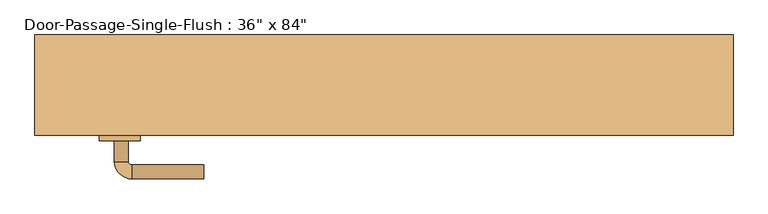
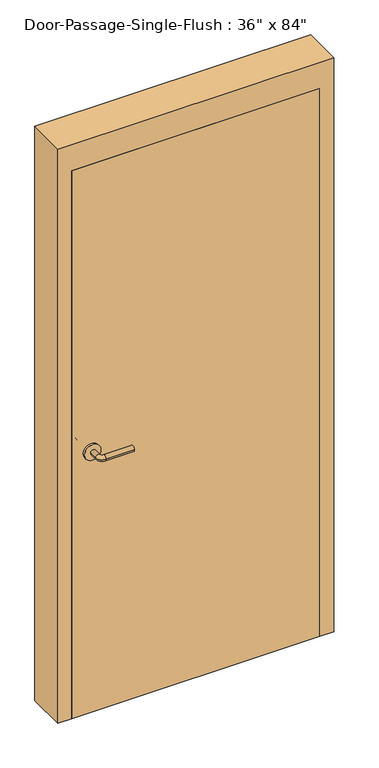
"""IFC4 building model written with IfcOpenShell, lengths in millimetres: door geometry."""

import ifcopenshell
import ifcopenshell.guid

model = None  # the IFC model being written
_history = None  # IfcOwnerHistory: only IFC2X3 demands one
_inside = {}  # id of a spatial element -> (the spatial element, [elements in it])
_under = {}  # id of a project, library or spatial element -> (it, [spatial elements below it])
_declared = {}  # id of a project -> (the project, [libraries it declares])
_typed = {}  # id of a type object -> (the type object, [elements of that type])
_made_of = {}  # id of a material, layer set ... -> (it, [elements and type objects made of it])


def new_model(schema):
    """Start an empty IFC model of exactly this schema.

    Asked for "IFC4X3", IfcOpenShell would pick the latest addendum, in which some entities
    have other attributes; the version numbers below select the first issue.
    IFC2X3 requires an IfcOwnerHistory on every rooted entity: one is made here for all.
    """
    global model, _history
    if schema == "IFC4X3":
        model = ifcopenshell.file(schema_version=(4, 3, 0, 0))
    else:
        model = ifcopenshell.file(schema=schema)
    _inside.clear()
    _under.clear()
    _declared.clear()
    _typed.clear()
    _made_of.clear()
    _history = None
    if model.schema == "IFC2X3":
        org = make("IfcOrganization", Name="unknown")
        user = make(
            "IfcPersonAndOrganization",
            ThePerson=make("IfcPerson", FamilyName="unknown"),
            TheOrganization=org,
        )
        app = make(
            "IfcApplication",
            ApplicationDeveloper=org,
            Version="unknown",
            ApplicationFullName="unknown",
            ApplicationIdentifier="unknown",
        )
        _history = make(
            "IfcOwnerHistory",
            OwningUser=user,
            OwningApplication=app,
            ChangeAction="ADDED",
            CreationDate=0,
        )
    return model


def make(cls, **values):
    """One entity of the class cls with the attributes given. An attribute that is None is left unset."""
    return model.create_entity(
        cls, **{name: value for name, value in values.items() if value is not None}
    )


def rooted(cls, **values):
    """An entity with a GlobalId (a new one), such as an element, a storey or a relation."""
    return make(cls, GlobalId=ifcopenshell.guid.new(), OwnerHistory=_history, **values)


def si_unit(unit_type, name, prefix=None):
    """IfcSIUnit, for example si_unit("LENGTHUNIT", "METRE", prefix="MILLI")."""
    return make("IfcSIUnit", UnitType=unit_type, Prefix=prefix, Name=name)


def assignment(units):
    """IfcUnitAssignment: the units of a project."""
    return None if units is None else make("IfcUnitAssignment", Units=units)


def point(xyz):
    """IfcCartesianPoint."""
    return None if xyz is None else make("IfcCartesianPoint", Coordinates=xyz)


def direction(xyz):
    """IfcDirection."""
    return None if xyz is None else make("IfcDirection", DirectionRatios=xyz)


def frame(location, z_axis=None, x_axis=None):
    """IfcAxis2Placement3D, a coordinate frame: its origin and axes. An axis left out is left unset."""
    return make(
        "IfcAxis2Placement3D",
        Location=point(location),
        Axis=direction(z_axis),
        RefDirection=direction(x_axis),
    )


def frame_2d(location, x_axis=None):
    """IfcAxis2Placement2D, a coordinate frame in the plane: its origin and x axis."""
    return make(
        "IfcAxis2Placement2D", Location=point(location), RefDirection=direction(x_axis)
    )


def origin():
    """The frame at (0, 0, 0) with its axes left unset."""
    return frame((0.0, 0.0, 0.0))


def origin_with_axes():
    """The frame at (0, 0, 0) with the z axis (0, 0, 1) and the x axis (1, 0, 0) written out."""
    return frame((0.0, 0.0, 0.0), z_axis=(0.0, 0.0, 1.0), x_axis=(1.0, 0.0, 0.0))


def place(relative_to, where):
    """IfcLocalPlacement: puts the frame where relative to a parent placement (None: the world)."""
    return make(
        "IfcLocalPlacement", PlacementRelTo=relative_to, RelativePlacement=where
    )


def context(
    kind, dimensions, precision=None, world=None, true_north=None, identifier=None
):
    """IfcGeometricRepresentationContext, for example the 3D "Model" context."""
    return make(
        "IfcGeometricRepresentationContext",
        ContextIdentifier=identifier,
        ContextType=kind,
        CoordinateSpaceDimension=dimensions,
        Precision=precision,
        WorldCoordinateSystem=world,
        TrueNorth=true_north,
    )


def project(units=None, contexts=None):
    """IfcProject with its units and contexts."""
    return rooted(
        "IfcProject",
        Name="project",
        RepresentationContexts=contexts,
        UnitsInContext=assignment(units),
    )


def spatial(cls, under=None, at=None, **own):
    """A site, building, storey or space (cls), placed at a placement, below another one or the project."""
    s = rooted(cls, ObjectPlacement=at, **own)
    if under is not None:
        _under.setdefault(under.id(), (under, []))[1].append(s)
    return s


def polyline(points):
    """IfcPolyline through the points."""
    return make("IfcPolyline", Points=[point(p) for p in points])


def circle_curve(where, radius):
    """IfcCircle in the frame where."""
    return make("IfcCircle", Position=where, Radius=radius)


def ellipse_curve(where, semi_axis1, semi_axis2):
    """IfcEllipse in the frame where."""
    return make(
        "IfcEllipse", Position=where, SemiAxis1=semi_axis1, SemiAxis2=semi_axis2
    )


def trimmed(basis, trim1, trim2, sense, master):
    """IfcTrimmedCurve: the piece of a basis curve between two trims."""
    return make(
        "IfcTrimmedCurve",
        BasisCurve=basis,
        Trim1=trim1,
        Trim2=trim2,
        SenseAgreement=sense,
        MasterRepresentation=master,
    )


def segment(curve, same_sense, transition):
    """IfcCompositeCurveSegment."""
    return make(
        "IfcCompositeCurveSegment",
        Transition=transition,
        SameSense=same_sense,
        ParentCurve=curve,
    )


def composite_curve(segments, self_intersect=None):
    """IfcCompositeCurve: segments joined end to end."""
    return make("IfcCompositeCurve", Segments=segments, SelfIntersect=self_intersect)


def outline(outer, holes=None, kind="AREA"):
    """IfcArbitraryClosedProfileDef: a profile drawn as a closed curve; with holes, ...WithVoids."""
    if holes is None:
        return make("IfcArbitraryClosedProfileDef", ProfileType=kind, OuterCurve=outer)
    return make(
        "IfcArbitraryProfileDefWithVoids",
        ProfileType=kind,
        OuterCurve=outer,
        InnerCurves=holes,
    )


def extrude(swept, where, along, depth):
    """IfcExtrudedAreaSolid: the profile swept, set in the frame where, extruded along a direction by depth."""
    return make(
        "IfcExtrudedAreaSolid",
        SweptArea=swept,
        Position=where,
        ExtrudedDirection=direction(along),
        Depth=depth,
    )


def faces_of(points, faces, orient=None, outer=None):
    """IfcFace entities. A face is a list of loops; a loop is a list of indices into points, from 0.

    orient and outer hold one flag for each loop. By default every Orientation is true, the
    first loop of a face is its IfcFaceOuterBound and the others are IfcFaceBound.
    """
    made = []
    for i, loops in enumerate(faces):
        bounds = []
        for j, loop in enumerate(loops):
            is_outer = j == 0 if outer is None else outer[i][j]
            bounds.append(
                make(
                    "IfcFaceOuterBound" if is_outer else "IfcFaceBound",
                    Bound=make("IfcPolyLoop", Polygon=[points[k] for k in loop]),
                    Orientation=True if orient is None else orient[i][j],
                )
            )
        made.append(make("IfcFace", Bounds=bounds))
    return made


def faceted_brep(points, faces, orient=None, outer=None, voids=None):
    """IfcFacetedBrep: a solid bounded by flat faces; with voids (closed shells), ...WithVoids."""
    shared = [point(p) for p in points]
    hull = make("IfcClosedShell", CfsFaces=faces_of(shared, faces, orient, outer))
    if voids is None:
        return make("IfcFacetedBrep", Outer=hull)
    return make(
        "IfcFacetedBrepWithVoids",
        Outer=hull,
        Voids=[
            make(cls, CfsFaces=faces_of(shared, fs, o, b)) for cls, fs, o, b in voids
        ],
    )


def shape(context_of_items, identifier, shape_type, items):
    """IfcShapeRepresentation: the items that make up one representation, for example the "Body"."""
    return make(
        "IfcShapeRepresentation",
        ContextOfItems=context_of_items,
        RepresentationIdentifier=identifier,
        RepresentationType=shape_type,
        Items=items,
    )


def source(mapping_origin, context_of_items, identifier, shape_type, items):
    """IfcRepresentationMap: a shape defined once, which mapped items show again and again."""
    return make(
        "IfcRepresentationMap",
        MappingOrigin=mapping_origin,
        MappedRepresentation=shape(context_of_items, identifier, shape_type, items),
    )


def transform(
    local_origin,
    x_axis=None,
    y_axis=None,
    z_axis=None,
    scale=None,
    scale2=None,
    scale3=None,
    uniform=True,
):
    """IfcCartesianTransformationOperator3D, or its non-uniform kind. x_axis, y_axis, z_axis: its Axis1, 2, 3."""
    if uniform:
        return make(
            "IfcCartesianTransformationOperator3D",
            Axis1=direction(x_axis),
            Axis2=direction(y_axis),
            LocalOrigin=point(local_origin),
            Scale=scale,
            Axis3=direction(z_axis),
        )
    return make(
        "IfcCartesianTransformationOperator3DnonUniform",
        Axis1=direction(x_axis),
        Axis2=direction(y_axis),
        LocalOrigin=point(local_origin),
        Scale=scale,
        Axis3=direction(z_axis),
        Scale2=scale2,
        Scale3=scale3,
    )


def mapped(mapping_source, mapping_target):
    """IfcMappedItem: shows the shape of a source again, moved by a transform."""
    return make(
        "IfcMappedItem", MappingSource=mapping_source, MappingTarget=mapping_target
    )


def made_of(thing, what):
    """Note that an element or type object is made of a material, layer set ...; save() writes the relation."""
    if what is not None:
        _made_of.setdefault(what.id(), (what, []))[1].append(thing)
    return thing


def element(
    cls,
    number,
    at=None,
    inside=None,
    cuts=None,
    type_object=None,
    material=None,
    context=None,
    identifier="Body",
    shape_type=None,
    held_by="IfcProductDefinitionShape",
    body=None,
    shapes=None,
    **own,
):
    """One element of the class cls, such as IfcWall. Its Tag is "e" and its number.

    at: its placement. inside: the storey or other place that contains it. cuts: it is an
    opening in that element (IfcRelVoidsElement). A single representation is given by context,
    identifier, shape_type and body (its items); several are given by shapes. held_by: the class
    of the entity that holds the representations. save() writes the other relations.
    """
    e = rooted(cls, Tag="e%d" % number, ObjectPlacement=at, **own)
    if body is not None:
        shapes = [shape(context, identifier, shape_type, body)]
    if shapes is not None:
        e.Representation = make(held_by, Representations=shapes)
    if inside is not None:
        _inside.setdefault(inside.id(), (inside, []))[1].append(e)
    if cuts is not None:
        rooted(
            "IfcRelVoidsElement", RelatingBuildingElement=cuts, RelatedOpeningElement=e
        )
    if type_object is not None:
        _typed.setdefault(type_object.id(), (type_object, []))[1].append(e)
    return made_of(e, material)


def aggregate(whole, parts):
    """IfcRelAggregates: a whole, such as a stair, and the parts it consists of."""
    return rooted("IfcRelAggregates", RelatingObject=whole, RelatedObjects=parts)


def save(model, path):
    """Write the relations noted so far, then the file.

    IfcRelAggregates (storeys below a building ...), IfcRelContainedInSpatialStructure (elements
    in a storey), IfcRelDefinesByType, IfcRelAssociatesMaterial and IfcRelDeclares: one each for
    every whole, place, type object, material and project.
    """
    for whole, parts in _under.values():
        aggregate(whole, parts)
    for where, things in _inside.values():
        rooted(
            "IfcRelContainedInSpatialStructure",
            RelatedElements=things,
            RelatingStructure=where,
        )
    for kind, things in _typed.values():
        rooted("IfcRelDefinesByType", RelatedObjects=things, RelatingType=kind)
    for what, things in _made_of.values():
        rooted("IfcRelAssociatesMaterial", RelatedObjects=things, RelatingMaterial=what)
    for by, libraries in _declared.values():
        rooted("IfcRelDeclares", RelatingContext=by, RelatedDefinitions=libraries)
    model.write(path)


def plane_surface(at):
    """IfcPlane: the flat surface through the origin of the frame at, square to its z axis."""
    return make("IfcPlane", Position=at)


def cylinder_surface(at, radius):
    """IfcCylindricalSurface: all points at the distance radius from the z axis of the frame at."""
    return make("IfcCylindricalSurface", Position=at, Radius=radius)


def revolved_surface(curve, axis_point, axis_direction):
    """IfcSurfaceOfRevolution: the curve turned about the line through axis_point along axis_direction."""
    return make(
        "IfcSurfaceOfRevolution",
        SweptCurve=make("IfcArbitraryOpenProfileDef", ProfileType="CURVE", Curve=curve),
        AxisPosition=make("IfcAxis1Placement", Location=point(axis_point), Axis=direction(axis_direction)),
    )


def advanced_brep(points, edges, surfaces, faces):
    """IfcAdvancedBrep: a solid bounded by faces that lie on surfaces and meet in shared edges.

    An edge is (start, end): straight between two places in points (the first is 0);
    or (start, end, curve); or (start, end, curve, False) where it runs against its curve.
    A face is (place in surfaces, loops), or (place, loops, False) where it looks against
    its surface's normal. A loop lists edges by number (the first is 1), with a minus sign
    where the edge is run from its end to its start. The first loop is the outer one.
    """
    corners = [point(p) for p in points]
    vertices = [make("IfcVertexPoint", VertexGeometry=c) for c in corners]
    made = []
    for start, end, *more in edges:
        made.append(
            make(
                "IfcEdgeCurve",
                EdgeStart=vertices[start],
                EdgeEnd=vertices[end],
                EdgeGeometry=more[0] if more else make("IfcPolyline", Points=[corners[start], corners[end]]),
                SameSense=more[1] if len(more) > 1 else True,
            )
        )
    hull = []
    for where, loops, *sense in faces:
        bounds = []
        for j, loop in enumerate(loops):
            ring = [make("IfcOrientedEdge", EdgeElement=made[abs(k) - 1], Orientation=k > 0) for k in loop]
            bounds.append(
                make(
                    "IfcFaceOuterBound" if j == 0 else "IfcFaceBound",
                    Bound=make("IfcEdgeLoop", EdgeList=ring),
                    Orientation=True,
                )
            )
        hull.append(make("IfcAdvancedFace", Bounds=bounds, FaceSurface=surfaces[where], SameSense=sense[0] if sense else True))
    return make("IfcAdvancedBrep", Outer=make("IfcClosedShell", CfsFaces=hull))


def door_36f17018(model_context):
    return source(origin(), model_context, "Body", "SolidModel", [
        advanced_brep(
        [(-392.190625, -23.75, 1016.0), (-372.190625, -23.75, 1016.0), (-392.190625, 6.25, 1016.0), (-372.190625, 6.25, 1016.0), (-367.190625, 11.25, 1016.0), (-367.190625, 31.25, 1016.0), (-262.190625, 31.25, 1016.0), (-262.190625, 11.25, 1016.0)],
        [
            (0, 1, circle_curve(frame((-382.190625, -23.75, 1016.0), z_axis=(0.0, -1.0, 0.0), x_axis=(1.0, 0.0, 0.0)), 10.0)),
            (1, 0, circle_curve(frame((-382.190625, -23.75, 1016.0), z_axis=(0.0, -1.0, 0.0), x_axis=(1.0, 0.0, 0.0)), 10.0)),
            (0, 2),
            (2, 3, circle_curve(frame((-382.190625, 6.25, 1016.0), z_axis=(0.0, -1.0, 0.0), x_axis=(1.0, 0.0, 0.0)), 10.0)),
            (3, 1),
            (3, 2, circle_curve(frame((-382.190625, 6.25, 1016.0), z_axis=(0.0, -1.0, 0.0), x_axis=(1.0, 0.0, 0.0)), 10.0)),
            (4, 3, circle_curve(frame((-367.190625, 6.25, 1016.0), z_axis=(0.0, 0.0, 1.0), x_axis=(-1.0, 0.0, 0.0)), 5.0)),
            (2, 5, circle_curve(frame((-367.190625, 6.25, 1016.0), z_axis=(0.0, 0.0, -1.0), x_axis=(-1.0, 0.0, 0.0)), 25.0)),
            (5, 4, circle_curve(frame((-367.190625, 21.25, 1016.0), z_axis=(-1.0, 0.0, 0.0), x_axis=(0.0, -1.0, 0.0)), 10.0)),
            (4, 5, circle_curve(frame((-367.190625, 21.25, 1016.0), z_axis=(-1.0, 0.0, 0.0), x_axis=(0.0, -1.0, 0.0)), 10.0)),
            (6, 7, circle_curve(frame((-262.190625, 21.25, 1016.0), z_axis=(1.0, 0.0, 0.0), x_axis=(0.0, -1.0, 0.0)), 10.0)),
            (7, 6, circle_curve(frame((-262.190625, 21.25, 1016.0), z_axis=(1.0, 0.0, 0.0), x_axis=(0.0, -1.0, 0.0)), 10.0)),
            (5, 6),
            (7, 4),
        ],
        [
            plane_surface(frame((-382.190625, -23.75, 1016.0), z_axis=(0.0, -1.0, 0.0), x_axis=(0.0, 0.0, 1.0))),
            cylinder_surface(frame((-382.190625, -23.75, 1016.0), z_axis=(0.0, -1.0, 0.0), x_axis=(1.0, 0.0, 0.0)), 10.0),
            revolved_surface(trimmed(ellipse_curve(frame((-382.190625, 6.25, 1016.0), z_axis=(0.0, -1.0, 0.0), x_axis=(1.0, 0.0, 0.0)), 10.0, 10.0), [point((-392.190625, 6.25, 1016.0))], [point((-372.190625, 6.25, 1016.0))], True, "CARTESIAN"), (-367.190625, 6.25, 1016.0), (0.0, 0.0, -1.0)),
            revolved_surface(trimmed(ellipse_curve(frame((-382.190625, 6.25, 1016.0), z_axis=(0.0, -1.0, 0.0), x_axis=(1.0, 0.0, 0.0)), 10.0, 10.0), [point((-372.190625, 6.25, 1016.0))], [point((-392.190625, 6.25, 1016.0))], True, "CARTESIAN"), (-367.190625, 6.25, 1016.0), (0.0, 0.0, -1.0)),
            plane_surface(frame((-262.190625, 21.25, 1016.0), z_axis=(1.0, 0.0, 0.0), x_axis=(0.0, 0.0, 1.0))),
            cylinder_surface(frame((-367.190625, 21.25, 1016.0), z_axis=(-1.0, 0.0, 0.0), x_axis=(0.0, -1.0, 0.0)), 10.0),
        ],
        [
            (0, [[1, 2]]),
            (1, [[-1, 3, 4, 5]]),
            (1, [[-2, -5, 6, -3]]),
            (2, [[7, -4, 8, 9]]),
            (3, [[-8, -6, -7, 10]]),
            (4, [[11, 12]]),
            (5, [[-9, 13, -12, 14]]),
            (5, [[-10, -14, -11, -13]]),
        ],
    ),
        extrude(outline(composite_curve([segment(trimmed(circle_curve(frame_2d((1016.0, -384.690625)), 30.0), [point((1016.0, -414.690625))], [point((1016.0, -354.690625))], False, "CARTESIAN"), True, "CONTINUOUS"), segment(trimmed(circle_curve(frame_2d((1016.0, -384.690625)), 30.0), [point((1016.0, -354.690625))], [point((1016.0, -414.690625))], False, "CARTESIAN"), True, "CONTINUOUS")], self_intersect=False)), frame((0.0, -31.75, 0.0), z_axis=(0.0, 1.0, 0.0), x_axis=(0.0, 0.0, 1.0)), (0.0, 0.0, 1.0), 8.0),
        advanced_brep(
        [(-392.190625, -84.2, 1016.0), (-372.190625, -84.2, 1016.0), (-372.190625, -114.2, 1016.0), (-392.190625, -114.2, 1016.0), (-367.190625, -119.2, 1016.0), (-367.190625, -139.2, 1016.0), (-262.190625, -139.2, 1016.0), (-262.190625, -119.2, 1016.0)],
        [
            (0, 1, circle_curve(frame((-382.190625, -84.2, 1016.0), z_axis=(0.0, 1.0, 0.0), x_axis=(1.0, 0.0, 0.0)), 10.0)),
            (1, 0, circle_curve(frame((-382.190625, -84.2, 1016.0), z_axis=(0.0, 1.0, 0.0), x_axis=(1.0, 0.0, 0.0)), 10.0)),
            (1, 2),
            (2, 3, circle_curve(frame((-382.190625, -114.2, 1016.0), z_axis=(0.0, 1.0, 0.0), x_axis=(1.0, 0.0, 0.0)), 10.0)),
            (3, 0),
            (3, 2, circle_curve(frame((-382.190625, -114.2, 1016.0), z_axis=(0.0, 1.0, 0.0), x_axis=(1.0, 0.0, 0.0)), 10.0)),
            (4, 5, circle_curve(frame((-367.190625, -129.2, 1016.0), z_axis=(-1.0, 0.0, 0.0), x_axis=(0.0, 1.0, 0.0)), 10.0)),
            (5, 3, circle_curve(frame((-367.190625, -114.2, 1016.0), z_axis=(0.0, 0.0, -1.0), x_axis=(-1.0, 0.0, 0.0)), 25.0)),
            (2, 4, circle_curve(frame((-367.190625, -114.2, 1016.0), z_axis=(0.0, 0.0, 1.0), x_axis=(-1.0, 0.0, 0.0)), 5.0)),
            (5, 4, circle_curve(frame((-367.190625, -129.2, 1016.0), z_axis=(-1.0, 0.0, 0.0), x_axis=(0.0, 1.0, 0.0)), 10.0)),
            (6, 7, circle_curve(frame((-262.190625, -129.2, 1016.0), z_axis=(1.0, 0.0, 0.0), x_axis=(0.0, 1.0, 0.0)), 10.0)),
            (7, 6, circle_curve(frame((-262.190625, -129.2, 1016.0), z_axis=(1.0, 0.0, 0.0), x_axis=(0.0, 1.0, 0.0)), 10.0)),
            (4, 7),
            (6, 5),
        ],
        [
            plane_surface(frame((-382.190625, -84.2, 1016.0), z_axis=(0.0, 1.0, 0.0), x_axis=(0.0, 0.0, 1.0))),
            cylinder_surface(frame((-382.190625, -84.2, 1016.0), z_axis=(0.0, 1.0, 0.0), x_axis=(1.0, 0.0, 0.0)), 10.0),
            revolved_surface(trimmed(ellipse_curve(frame((-382.190625, -114.2, 1016.0), z_axis=(0.0, -1.0, 0.0), x_axis=(1.0, 0.0, 0.0)), 10.0, 10.0), [point((-392.190625, -114.2, 1016.0))], [point((-372.190625, -114.2, 1016.0))], True, "CARTESIAN"), (-367.190625, -114.2, 1016.0), (0.0, 0.0, -1.0)),
            revolved_surface(trimmed(ellipse_curve(frame((-382.190625, -114.2, 1016.0), z_axis=(0.0, -1.0, 0.0), x_axis=(1.0, 0.0, 0.0)), 10.0, 10.0), [point((-372.190625, -114.2, 1016.0))], [point((-392.190625, -114.2, 1016.0))], True, "CARTESIAN"), (-367.190625, -114.2, 1016.0), (0.0, 0.0, -1.0)),
            plane_surface(frame((-262.190625, -129.2, 1016.0), z_axis=(1.0, 0.0, 0.0), x_axis=(0.0, 0.0, 1.0))),
            cylinder_surface(frame((-367.190625, -129.2, 1016.0), z_axis=(-1.0, 0.0, 0.0), x_axis=(0.0, 1.0, 0.0)), 10.0),
        ],
        [
            (0, [[1, 2]]),
            (1, [[3, 4, 5, -2]]),
            (1, [[-5, 6, -3, -1]]),
            (2, [[7, 8, -4, 9]]),
            (3, [[10, -9, -6, -8]]),
            (4, [[11, 12]]),
            (5, [[13, -11, 14, -7]]),
            (5, [[-14, -12, -13, -10]]),
        ],
    ),
        extrude(outline(composite_curve([segment(trimmed(circle_curve(frame_2d((1016.0, -384.690625)), 30.0), [point((1016.0, -414.690625))], [point((1016.0, -354.690625))], False, "CARTESIAN"), True, "CONTINUOUS"), segment(trimmed(circle_curve(frame_2d((1016.0, -384.690625)), 30.0), [point((1016.0, -354.690625))], [point((1016.0, -414.690625))], False, "CARTESIAN"), True, "CONTINUOUS")], self_intersect=False)), frame((0.0, -84.2, 0.0), z_axis=(0.0, 1.0, 0.0), x_axis=(0.0, 0.0, 1.0)), (0.0, 0.0, 1.0), 8.0),
        faceted_brep([(457.2, -26.9875, 0.0), (441.325, -26.9875, 0.0), (441.325, 20.6375, 0.0), (457.2, 20.6375, 0.0), (457.2, 69.85, 0.0), (508.0, 69.85, 0.0), (508.0, -76.2, 0.0), (457.2, -76.2, 0.0), (457.2, -76.2, 2133.6), (457.2, -26.9875, 2133.6), (508.0, -76.2, 2235.2), (-508.0, -76.2, 2235.2), (-508.0, -76.2, 0.0), (-457.2, -76.2, 0.0), (-457.2, -76.2, 2133.6), (508.0, 69.85, 2235.2), (457.2, 69.85, 2133.6), (-457.2, 69.85, 2133.6), (-457.2, 69.85, 0.0), (-508.0, 69.85, 0.0), (-508.0, 69.85, 2235.2), (457.2, 20.6375, 2133.6), (441.325, 20.6375, 2117.725), (-441.325, 20.6375, 2117.725), (-441.325, 20.6375, 0.0), (-457.2, 20.6375, 0.0), (-457.2, 20.6375, 2133.6), (441.325, -26.9875, 2117.725), (-457.2, -26.9875, 2133.6), (-457.2, -26.9875, 0.0), (-441.325, -26.9875, 0.0), (-441.325, -26.9875, 2117.725)], [[[0, 1, 2, 3, 4, 5, 6, 7]], [[7, 8, 9, 0]], [[6, 10, 11, 12, 13, 14, 8, 7]], [[5, 15, 10, 6]], [[4, 16, 17, 18, 19, 20, 15, 5]], [[3, 21, 16, 4]], [[2, 22, 23, 24, 25, 26, 21, 3]], [[1, 27, 22, 2]], [[0, 9, 28, 29, 30, 31, 27, 1]], [[8, 14, 28, 9]], [[16, 21, 26, 17]], [[22, 27, 31, 23]], [[12, 19, 18, 25, 24, 30, 29, 13]], [[13, 29, 28, 14]], [[11, 20, 19, 12]], [[17, 26, 25, 18]], [[23, 31, 30, 24]], [[15, 20, 11, 10]]]),
        extrude(outline(polyline([(457.2, -31.75), (457.2, -76.2), (-457.2, -76.2), (-457.2, -31.75), (457.2, -31.75)])), origin_with_axes(), (0.0, 0.0, 1.0), 2133.6),
    ])


if __name__ == "__main__":
    model = new_model("IFC4")
    model_context = context("Model", 3, world=origin())
    ifc_project = project(units=[si_unit("LENGTHUNIT", "METRE", prefix="MILLI")], contexts=[model_context])
    site = spatial("IfcSite", under=ifc_project)
    building = spatial("IfcBuilding", under=site)
    placement = place(None, origin())
    door_shape = door_36f17018(model_context)
    element("IfcDoor", 1, ObjectType="Door-Passage-Single-Flush : 36\" x 84\"", at=placement, inside=building, context=model_context, shape_type="MappedRepresentation", body=[
        mapped(door_shape, transform((0.0, 0.0, 0.0), x_axis=(1.0, 0.0, 0.0), y_axis=(0.0, 1.0, 0.0), z_axis=(0.0, 0.0, 1.0))),
    ])
    save(model, "model.ifc")

# Revit data of these elements
# Type "Door-Passage-Single-Flush : 36\" x 84\""
#   Type Mark = "35"
#   Assembly Code = "B2030200"
#   Analytic Construction = "Wooden"
#   Thickness = 0' - 1 3/4"
#   Thermal Resistance (R) = 2.5876 (h·ft²·°F)/BTU
#   Swing Angle [instance default] = 90.00°
#   Strike Height = 3' - 4"
#   Rough Width [instance default] = 3' - 4"
#   Rough Height [instance default] = 7' - 4"
#   MF Opening Height [instance default] = 0' - 4"
#   MF Opening Width [instance default] = 0' - 4"
#   Inset Calculate [instance default] = 0' - 4"
#   Masonry Inset [instance default] = 0' - 1"
#   Height = 7' - 0"
#   Width = 3' - 0"
#   Heat Transfer Coefficient (U) = 0.3865 BTU/(h·ft²·°F)
#   Masonry Frame Depth = 0' - 5 3/4"
#   Masonry Frame [instance default] = yes
#   Function = 1
#   Dry Wall Frame [instance default] = no
#   Panel Material = Wood - Birch
#   Frame Material = Metal - Paint Finish - Grey
#   Door Handle Material = Aluminum
#   Visual Light Transmittance = 0
#   Solar Heat Gain Coefficient = 0
#   Wall Closure = (empty or 0)
# Element 1 (IfcDoor, "Door-Passage-Single-Flush : 36\" x 84\"")
#   Inset Calculate = 0' - 3"
#   Masonry Inset = 0' - 0"
#   Materials on its faces: "Aluminum", "Metal - Paint Finish - Grey", "Wood - Birch"
# Materials
#   "Wood - Birch": class "Wood", colour RGB 166 116 52, transparency 0, Cost = 0
#   "Metal - Paint Finish - Grey": class "Paint", colour RGB 104 104 104, transparency 0, Cost = 0
#   "Aluminum": class "Metal", colour RGB 247 247 247, transparency 0, Description = "Aluminum 6061", Cost = 0
